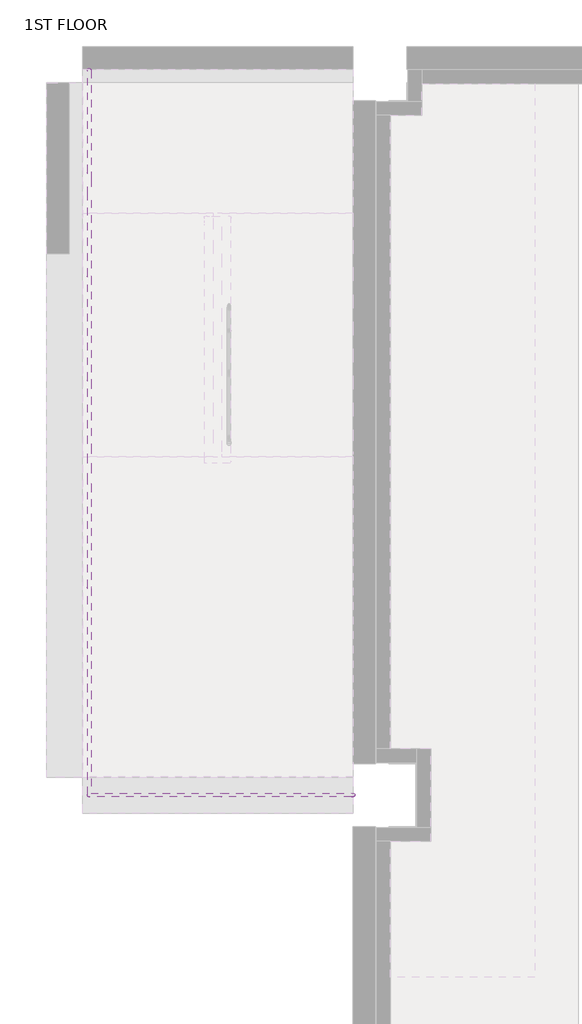
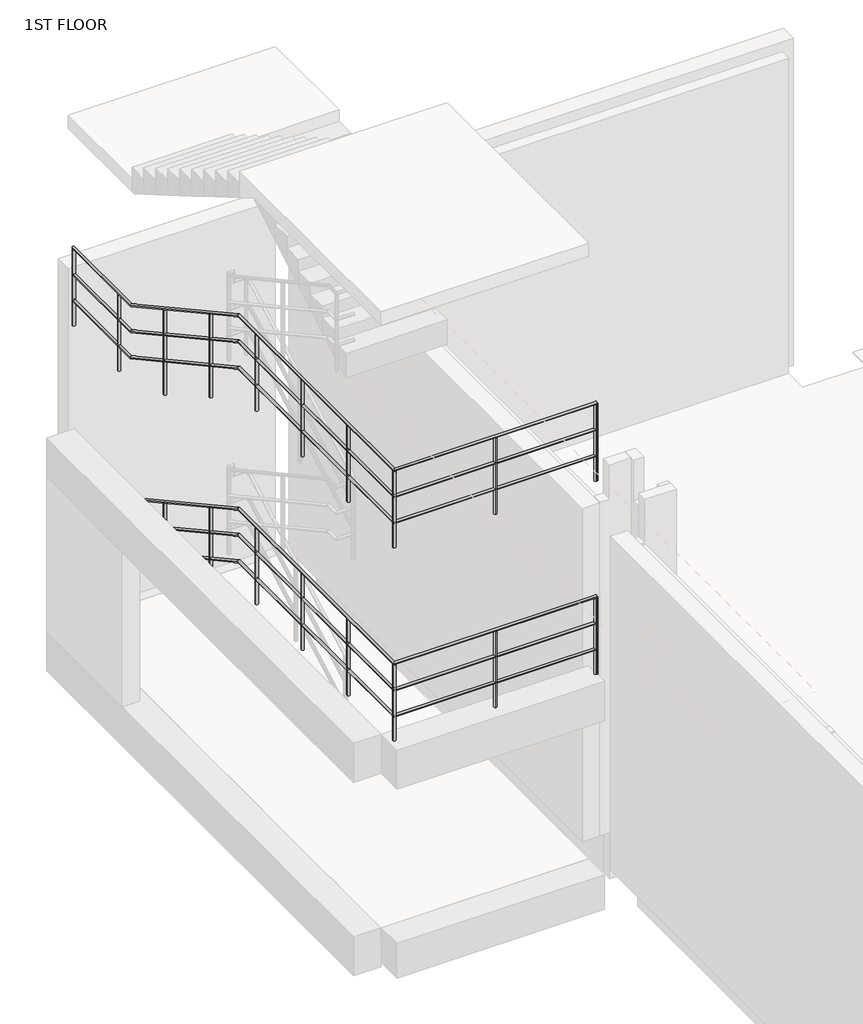
# One storey, part 11 of 15: 2 railings.
"""IFC4 building model written with IfcOpenShell, lengths in millimetres."""

from ifc_helpers import new_model, si_unit, point, frame, frame_2d, origin, place, context, project, spatial, circle_curve, ellipse_curve, trimmed, segment, composite_curve, outline, extrude, element, save
from ifc_brep_helpers import plane_surface, cylinder_surface, advanced_brep

model = new_model("IFC4")

# Units and contexts
model_context = context("Model", 3, world=origin())
ifc_project = project(units=[si_unit("LENGTHUNIT", "METRE", prefix="MILLI")], contexts=[model_context])

# Site, building, storey
site = spatial("IfcSite", under=ifc_project)
building = spatial("IfcBuilding", under=site)
storey = spatial("IfcBuildingStorey", under=building, Name="1ST FLOOR", Elevation=4800.0)

# Railings
placement = place(None, origin())
element("IfcRailing", 1, ObjectType="H_RL_AR_S10_Steel Handrail_H1200_STAIR", at=placement, inside=storey, context=model_context, shape_type="SolidModel", body=[
    advanced_brep(
    [(-3244.0, 50.0, 7291.0), (-3206.0, 50.0, 7291.0), (-3244.0, -1404.865872, 7291.0), (-3206.0, -1404.865872, 7291.0), (-300.0, -8019.0, 8771.0), (-300.0, -7981.0, 8771.0), (-3206.0, -7981.0, 8771.0), (-3244.0, -8019.0, 8771.0), (-3244.0, -4104.865872, 8771.0), (-3206.0, -4104.865872, 8771.0)],
    [
        (0, 1, circle_curve(frame((-3225.0, 50.0, 7291.0), z_axis=(0.0, 1.0, 0.0), x_axis=(1.0, 0.0, 0.0)), 19.0)),
        (1, 0, circle_curve(frame((-3225.0, 50.0, 7291.0), z_axis=(0.0, 1.0, 0.0), x_axis=(1.0, 0.0, 0.0)), 19.0)),
        (0, 2),
        (2, 3, ellipse_curve(frame((-3225.0, -1404.865872, 7291.0), z_axis=(0.0, 0.968736479519294, -0.24809198545814548), x_axis=(0.0, 0.24809198545814504, 0.9687364795192941)), 19.613177, 19.0)),
        (3, 1),
        (3, 2, ellipse_curve(frame((-3225.0, -1404.865872, 7291.0), z_axis=(0.0, 0.968736479519294, -0.24809198545814548), x_axis=(0.0, 0.24809198545814504, 0.9687364795192941)), 19.613177, 19.0)),
        (4, 5, circle_curve(frame((-300.0, -8000.0, 8771.0), z_axis=(1.0, 0.0, 0.0), x_axis=(0.0, 1.0, 0.0)), 19.0)),
        (5, 4, circle_curve(frame((-300.0, -8000.0, 8771.0), z_axis=(1.0, 0.0, 0.0), x_axis=(0.0, 1.0, 0.0)), 19.0)),
        (6, 7, ellipse_curve(frame((-3225.0, -8000.0, 8771.0), z_axis=(0.7071067811865469, -0.707106781186548, 0.0), x_axis=(-0.7071067811865481, -0.7071067811865468, 0.0)), 26.8700577, 19.0)),
        (7, 4),
        (5, 6),
        (7, 6, ellipse_curve(frame((-3225.0, -8000.0, 8771.0), z_axis=(0.7071067811865469, -0.707106781186548, 0.0), x_axis=(-0.7071067811865481, -0.7071067811865468, 0.0)), 26.8700577, 19.0)),
        (2, 8),
        (8, 9, ellipse_curve(frame((-3225.0, -4104.865872, 8771.0), z_axis=(0.0, 0.968736479519294, -0.24809198545814548), x_axis=(0.0, -0.24809198545814592, -0.9687364795192939)), 19.613177, 19.0)),
        (9, 3),
        (9, 8, ellipse_curve(frame((-3225.0, -4104.865872, 8771.0), z_axis=(0.0, 0.968736479519294, -0.24809198545814548), x_axis=(0.0, -0.24809198545814592, -0.9687364795192939)), 19.613177, 19.0)),
        (8, 7),
        (6, 9),
    ],
    [
        plane_surface(frame((-3225.0, 50.0, 7310.0), z_axis=(0.0, 1.0, 0.0), x_axis=(0.0, 0.0, -1.0))),
        cylinder_surface(frame((-3225.0, 50.0, 7291.0), z_axis=(0.0, 1.0, 0.0), x_axis=(1.0, 0.0, 0.0)), 19.0),
        plane_surface(frame((-300.0, -8000.0, 8790.0), z_axis=(1.0, 0.0, 0.0), x_axis=(0.0, 1.0, 0.0))),
        cylinder_surface(frame((-3225.0, -8000.0, 8771.0), z_axis=(-1.0, 0.0, 0.0), x_axis=(0.0, 1.0, 0.0)), 19.0),
        cylinder_surface(frame((-3225.0, -1409.1327588, 7293.3388861), z_axis=(0.0, 0.8769007335028707, -0.4806715131793514), x_axis=(1.0, 0.0, 0.0)), 19.0),
        cylinder_surface(frame((-3225.0, -4100.0, 8771.0), z_axis=(0.0, 1.0, 0.0), x_axis=(1.0, 0.0, 0.0)), 19.0),
    ],
    [
        (0, [[1, 2]]),
        (1, [[-1, 3, 4, 5]]),
        (1, [[-2, -5, 6, -3]]),
        (2, [[7, 8]]),
        (3, [[9, 10, -8, 11]]),
        (3, [[12, -11, -7, -10]]),
        (4, [[-4, 13, 14, 15]]),
        (4, [[-6, -15, 16, -13]]),
        (5, [[-14, 17, -9, 18]]),
        (5, [[-16, -18, -12, -17]]),
    ],
),
    advanced_brep(
    [(-3206.0, 50.0, 6491.0), (-3244.0, 50.0, 6491.0), (-3206.0, -1404.865872, 6491.0), (-3244.0, -1404.865872, 6491.0), (-3206.0, -4104.865872, 7971.0), (-3244.0, -4104.865872, 7971.0), (-3206.0, -7981.0, 7971.0), (-3244.0, -8019.0, 7971.0)],
    [
        (0, 1, circle_curve(frame((-3225.0, 50.0, 6491.0), z_axis=(0.0, 1.0, 0.0), x_axis=(-1.0, 0.0, 0.0)), 19.0)),
        (1, 0, circle_curve(frame((-3225.0, 50.0, 6491.0), z_axis=(0.0, 1.0, 0.0), x_axis=(-1.0, 0.0, 0.0)), 19.0)),
        (0, 2),
        (2, 3, ellipse_curve(frame((-3225.0, -1404.865872, 6491.0), z_axis=(0.0, 0.968736479519294, -0.24809198545814548), x_axis=(0.0, 0.24809198545814504, 0.9687364795192941)), 19.613177, 19.0)),
        (3, 1),
        (3, 2, ellipse_curve(frame((-3225.0, -1404.865872, 6491.0), z_axis=(0.0, 0.968736479519294, -0.24809198545814548), x_axis=(0.0, 0.24809198545814504, 0.9687364795192941)), 19.613177, 19.0)),
        (2, 4),
        (4, 5, ellipse_curve(frame((-3225.0, -4104.865872, 7971.0), z_axis=(0.0, 0.968736479519294, -0.24809198545814548), x_axis=(0.0, -0.24809198545814592, -0.9687364795192939)), 19.613177, 19.0)),
        (5, 3),
        (5, 4, ellipse_curve(frame((-3225.0, -4104.865872, 7971.0), z_axis=(0.0, 0.968736479519294, -0.24809198545814548), x_axis=(0.0, -0.24809198545814592, -0.9687364795192939)), 19.613177, 19.0)),
        (6, 7, ellipse_curve(frame((-3225.0, -8000.0, 7971.0), z_axis=(0.7071067811865464, -0.7071067811865487, 0.0), x_axis=(0.7071067811865487, 0.7071067811865464, 0.0)), 26.8700577, 19.0)),
        (7, 6, ellipse_curve(frame((-3225.0, -8000.0, 7971.0), z_axis=(0.7071067811865464, -0.7071067811865487, 0.0), x_axis=(0.7071067811865487, 0.7071067811865464, 0.0)), 26.8700577, 19.0)),
        (4, 6),
        (7, 5),
    ],
    [
        plane_surface(frame((-3225.0, 50.0, 6510.0), z_axis=(0.0, 1.0, 0.0), x_axis=(0.0, 0.0, -1.0))),
        cylinder_surface(frame((-3225.0, 50.0, 6491.0), z_axis=(0.0, 1.0, 0.0), x_axis=(-1.0, 0.0, 0.0)), 19.0),
        cylinder_surface(frame((-3225.0, -1409.1327588, 6493.3388861), z_axis=(0.0, 0.8769007335028707, -0.4806715131793514), x_axis=(-1.0, 0.0, 0.0)), 19.0),
        plane_surface(frame((-3225.0, -8000.0, 7990.0), z_axis=(0.7071067811865464, -0.7071067811865487, 0.0), x_axis=(0.7071067811865487, 0.7071067811865464, 0.0))),
        cylinder_surface(frame((-3225.0, -4100.0, 7971.0), z_axis=(0.0, 1.0, 0.0), x_axis=(-1.0, 0.0, 0.0)), 19.0),
    ],
    [
        (0, [[1, 2]]),
        (1, [[-1, 3, 4, 5]]),
        (1, [[-2, -5, 6, -3]]),
        (2, [[-4, 7, 8, 9]]),
        (2, [[-6, -9, 10, -7]]),
        (3, [[11, 12]]),
        (4, [[-8, 13, -12, 14]]),
        (4, [[-10, -14, -11, -13]]),
    ],
),
    advanced_brep(
    [(-3206.0, -7981.0, 7971.0), (-3244.0, -8019.0, 7971.0), (-300.0, -7981.0, 7971.0), (-300.0, -8019.0, 7971.0)],
    [
        (0, 1, ellipse_curve(frame((-3225.0, -8000.0, 7971.0), z_axis=(-0.7071067811865464, 0.7071067811865487, 0.0), x_axis=(-0.7071067811865487, -0.7071067811865464, 0.0)), 26.8700577, 19.0)),
        (1, 0, ellipse_curve(frame((-3225.0, -8000.0, 7971.0), z_axis=(-0.7071067811865464, 0.7071067811865487, 0.0), x_axis=(-0.7071067811865487, -0.7071067811865464, 0.0)), 26.8700577, 19.0)),
        (2, 3, circle_curve(frame((-300.0, -8000.0, 7971.0), z_axis=(1.0, 0.0, 0.0), x_axis=(0.0, -1.0, 0.0)), 19.0)),
        (3, 2, circle_curve(frame((-300.0, -8000.0, 7971.0), z_axis=(1.0, 0.0, 0.0), x_axis=(0.0, -1.0, 0.0)), 19.0)),
        (0, 2),
        (3, 1),
    ],
    [
        plane_surface(frame((-3225.0, -8000.0, 7990.0), z_axis=(-0.7071067811865464, 0.7071067811865487, 0.0), x_axis=(0.7071067811865487, 0.7071067811865464, 0.0))),
        plane_surface(frame((-300.0, -8000.0, 7990.0), z_axis=(1.0, 0.0, 0.0), x_axis=(0.0, 1.0, 0.0))),
        cylinder_surface(frame((-3225.0, -8000.0, 7971.0), z_axis=(-1.0, 0.0, 0.0), x_axis=(0.0, -1.0, 0.0)), 19.0),
    ],
    [
        (0, [[1, 2]]),
        (1, [[3, 4]]),
        (2, [[-1, 5, -4, 6]]),
        (2, [[-2, -6, -3, -5]]),
    ],
),
    advanced_brep(
    [(-3206.0, 50.0, 6891.0), (-3244.0, 50.0, 6891.0), (-3206.0, -1404.865872, 6891.0), (-3244.0, -1404.865872, 6891.0), (-3206.0, -4104.865872, 8371.0), (-3244.0, -4104.865872, 8371.0), (-3206.0, -7981.0, 8371.0), (-3244.0, -8019.0, 8371.0)],
    [
        (0, 1, circle_curve(frame((-3225.0, 50.0, 6891.0), z_axis=(0.0, 1.0, 0.0), x_axis=(-1.0, 0.0, 0.0)), 19.0)),
        (1, 0, circle_curve(frame((-3225.0, 50.0, 6891.0), z_axis=(0.0, 1.0, 0.0), x_axis=(-1.0, 0.0, 0.0)), 19.0)),
        (0, 2),
        (2, 3, ellipse_curve(frame((-3225.0, -1404.865872, 6891.0), z_axis=(0.0, 0.968736479519294, -0.24809198545814548), x_axis=(0.0, 0.24809198545814504, 0.9687364795192941)), 19.613177, 19.0)),
        (3, 1),
        (3, 2, ellipse_curve(frame((-3225.0, -1404.865872, 6891.0), z_axis=(0.0, 0.968736479519294, -0.24809198545814548), x_axis=(0.0, 0.24809198545814504, 0.9687364795192941)), 19.613177, 19.0)),
        (2, 4),
        (4, 5, ellipse_curve(frame((-3225.0, -4104.865872, 8371.0), z_axis=(0.0, 0.968736479519294, -0.24809198545814548), x_axis=(0.0, -0.24809198545814592, -0.9687364795192939)), 19.613177, 19.0)),
        (5, 3),
        (5, 4, ellipse_curve(frame((-3225.0, -4104.865872, 8371.0), z_axis=(0.0, 0.968736479519294, -0.24809198545814548), x_axis=(0.0, -0.24809198545814592, -0.9687364795192939)), 19.613177, 19.0)),
        (6, 7, ellipse_curve(frame((-3225.0, -8000.0, 8371.0), z_axis=(0.7071067811865464, -0.7071067811865487, 0.0), x_axis=(0.7071067811865487, 0.7071067811865464, 0.0)), 26.8700577, 19.0)),
        (7, 6, ellipse_curve(frame((-3225.0, -8000.0, 8371.0), z_axis=(0.7071067811865464, -0.7071067811865487, 0.0), x_axis=(0.7071067811865487, 0.7071067811865464, 0.0)), 26.8700577, 19.0)),
        (4, 6),
        (7, 5),
    ],
    [
        plane_surface(frame((-3225.0, 50.0, 6910.0), z_axis=(0.0, 1.0, 0.0), x_axis=(0.0, 0.0, -1.0))),
        cylinder_surface(frame((-3225.0, 50.0, 6891.0), z_axis=(0.0, 1.0, 0.0), x_axis=(-1.0, 0.0, 0.0)), 19.0),
        cylinder_surface(frame((-3225.0, -1409.1327588, 6893.3388861), z_axis=(0.0, 0.8769007335028707, -0.4806715131793514), x_axis=(-1.0, 0.0, 0.0)), 19.0),
        plane_surface(frame((-3225.0, -8000.0, 8390.0), z_axis=(0.7071067811865464, -0.7071067811865487, 0.0), x_axis=(0.7071067811865487, 0.7071067811865464, 0.0))),
        cylinder_surface(frame((-3225.0, -4100.0, 8371.0), z_axis=(0.0, 1.0, 0.0), x_axis=(-1.0, 0.0, 0.0)), 19.0),
    ],
    [
        (0, [[1, 2]]),
        (1, [[-1, 3, 4, 5]]),
        (1, [[-2, -5, 6, -3]]),
        (2, [[-4, 7, 8, 9]]),
        (2, [[-6, -9, 10, -7]]),
        (3, [[11, 12]]),
        (4, [[-8, 13, -12, 14]]),
        (4, [[-10, -14, -11, -13]]),
    ],
),
    advanced_brep(
    [(-3206.0, -7981.0, 8371.0), (-3244.0, -8019.0, 8371.0), (-300.0, -7981.0, 8371.0), (-300.0, -8019.0, 8371.0)],
    [
        (0, 1, ellipse_curve(frame((-3225.0, -8000.0, 8371.0), z_axis=(-0.7071067811865464, 0.7071067811865487, 0.0), x_axis=(-0.7071067811865487, -0.7071067811865464, 0.0)), 26.8700577, 19.0)),
        (1, 0, ellipse_curve(frame((-3225.0, -8000.0, 8371.0), z_axis=(-0.7071067811865464, 0.7071067811865487, 0.0), x_axis=(-0.7071067811865487, -0.7071067811865464, 0.0)), 26.8700577, 19.0)),
        (2, 3, circle_curve(frame((-300.0, -8000.0, 8371.0), z_axis=(1.0, 0.0, 0.0), x_axis=(0.0, -1.0, 0.0)), 19.0)),
        (3, 2, circle_curve(frame((-300.0, -8000.0, 8371.0), z_axis=(1.0, 0.0, 0.0), x_axis=(0.0, -1.0, 0.0)), 19.0)),
        (0, 2),
        (3, 1),
    ],
    [
        plane_surface(frame((-3225.0, -8000.0, 8390.0), z_axis=(-0.7071067811865464, 0.7071067811865487, 0.0), x_axis=(0.7071067811865487, 0.7071067811865464, 0.0))),
        plane_surface(frame((-300.0, -8000.0, 8390.0), z_axis=(1.0, 0.0, 0.0), x_axis=(0.0, 1.0, 0.0))),
        cylinder_surface(frame((-3225.0, -8000.0, 8371.0), z_axis=(-1.0, 0.0, 0.0), x_axis=(0.0, -1.0, 0.0)), 19.0),
    ],
    [
        (0, [[1, 2]]),
        (1, [[3, 4]]),
        (2, [[-1, 5, -4, 6]]),
        (2, [[-2, -6, -3, -5]]),
    ],
),
    extrude(outline(composite_curve([segment(trimmed(circle_curve(frame_2d((-300.0, -8000.0)), 21.2), [point((-300.0, -7978.8))], [point((-300.0, -8021.2))], False, "CARTESIAN"), True, "CONTINUOUS"), segment(trimmed(circle_curve(frame_2d((-300.0, -8000.0)), 21.2), [point((-300.0, -8021.2))], [point((-300.0, -7978.8))], False, "CARTESIAN"), True, "CONTINUOUS")], self_intersect=False)), frame((0.0, 0.0, 7590.0), z_axis=(0.0, 0.0, 1.0), x_axis=(1.0, 0.0, 0.0)), (0.0, 0.0, 1.0), 1162.0),
    extrude(outline(composite_curve([segment(trimmed(circle_curve(frame_2d((-1762.5, -8000.0)), 21.2), [point((-1762.5, -7978.8))], [point((-1762.5, -8021.2))], False, "CARTESIAN"), True, "CONTINUOUS"), segment(trimmed(circle_curve(frame_2d((-1762.5, -8000.0)), 21.2), [point((-1762.5, -8021.2))], [point((-1762.5, -7978.8))], False, "CARTESIAN"), True, "CONTINUOUS")], self_intersect=False)), frame((0.0, 0.0, 7590.0), z_axis=(0.0, 0.0, 1.0), x_axis=(1.0, 0.0, 0.0)), (0.0, 0.0, 1.0), 1162.0),
    extrude(outline(composite_curve([segment(trimmed(circle_curve(frame_2d((-3225.0, -8000.0)), 21.2), [point((-3203.8, -8000.0))], [point((-3246.2, -8000.0))], False, "CARTESIAN"), True, "CONTINUOUS"), segment(trimmed(circle_curve(frame_2d((-3225.0, -8000.0)), 21.2), [point((-3246.2, -8000.0))], [point((-3203.8, -8000.0))], False, "CARTESIAN"), True, "CONTINUOUS")], self_intersect=False)), frame((0.0, 0.0, 7590.0), z_axis=(0.0, 0.0, 1.0), x_axis=(1.0, 0.0, 0.0)), (0.0, 0.0, 1.0), 1162.0),
    extrude(outline(composite_curve([segment(trimmed(circle_curve(frame_2d((-3225.0, -6850.0)), 21.2), [point((-3203.8, -6850.0))], [point((-3246.2, -6850.0))], False, "CARTESIAN"), True, "CONTINUOUS"), segment(trimmed(circle_curve(frame_2d((-3225.0, -6850.0)), 21.2), [point((-3246.2, -6850.0))], [point((-3203.8, -6850.0))], False, "CARTESIAN"), True, "CONTINUOUS")], self_intersect=False)), frame((0.0, 0.0, 7590.0), z_axis=(0.0, 0.0, 1.0), x_axis=(1.0, 0.0, 0.0)), (0.0, 0.0, 1.0), 1162.0),
    extrude(outline(composite_curve([segment(trimmed(circle_curve(frame_2d((-3225.0, -5700.0)), 21.2), [point((-3203.8, -5700.0))], [point((-3246.2, -5700.0))], False, "CARTESIAN"), True, "CONTINUOUS"), segment(trimmed(circle_curve(frame_2d((-3225.0, -5700.0)), 21.2), [point((-3246.2, -5700.0))], [point((-3203.8, -5700.0))], False, "CARTESIAN"), True, "CONTINUOUS")], self_intersect=False)), frame((0.0, 0.0, 7590.0), z_axis=(0.0, 0.0, 1.0), x_axis=(1.0, 0.0, 0.0)), (0.0, 0.0, 1.0), 1162.0),
    extrude(outline(composite_curve([segment(trimmed(circle_curve(frame_2d((-3225.0, -4550.0)), 21.2), [point((-3203.8, -4550.0))], [point((-3246.2, -4550.0))], False, "CARTESIAN"), True, "CONTINUOUS"), segment(trimmed(circle_curve(frame_2d((-3225.0, -4550.0)), 21.2), [point((-3246.2, -4550.0))], [point((-3203.8, -4550.0))], False, "CARTESIAN"), True, "CONTINUOUS")], self_intersect=False)), frame((0.0, 0.0, 7590.0), z_axis=(0.0, 0.0, 1.0), x_axis=(1.0, 0.0, 0.0)), (0.0, 0.0, 1.0), 1162.0),
    advanced_brep(
    [(-3246.2, -3400.0, 8362.9618588), (-3246.2, -3400.0, 7096.6666667), (-3203.8, -3400.0, 7096.6666667), (-3203.8, -3400.0, 8362.9618588)],
    [
        (0, 1),
        (1, 2, circle_curve(frame((-3225.0, -3400.0, 7096.6666667), z_axis=(0.0, 0.0, 1.0), x_axis=(1.0, 0.0, 0.0)), 21.2)),
        (2, 3),
        (3, 0, ellipse_curve(frame((-3225.0, -3400.0, 8362.9618588), z_axis=(0.0, -0.4806715131793532, -0.8769007335028697), x_axis=(0.0, -0.8769007335028696, 0.4806715131793532)), 24.1760546, 21.2)),
        (0, 3, ellipse_curve(frame((-3225.0, -3400.0, 8362.9618588), z_axis=(0.0, -0.4806715131793532, -0.8769007335028697), x_axis=(0.0, -0.8769007335028696, 0.4806715131793532)), 24.1760546, 21.2)),
        (2, 1, circle_curve(frame((-3225.0, -3400.0, 7096.6666667), z_axis=(0.0, 0.0, 1.0), x_axis=(1.0, 0.0, 0.0)), 21.2)),
    ],
    [
        cylinder_surface(frame((-3225.0, -3400.0, 6996.6666667), z_axis=(0.0, 0.0, 1.0), x_axis=(1.0, 0.0, 0.0)), 21.2),
        plane_surface(frame((-3200.0, -3425.0, 8376.6655625), z_axis=(0.0, 0.4806715131793532, 0.8769007335028697), x_axis=(-1.0, 0.0, 0.0))),
        plane_surface(frame((-3200.0, -3375.0, 7096.6666667), z_axis=(0.0, 0.0, -1.0), x_axis=(-1.0, 0.0, 0.0))),
    ],
    [
        (0, [[1, 2, 3, 4]]),
        (0, [[-1, 5, -3, 6]]),
        (1, [[-4, -5]]),
        (2, [[-2, -6]]),
    ],
),
    advanced_brep(
    [(-3246.2, -2250.0, 7732.5914885), (-3246.2, -2250.0, 6438.8888889), (-3203.8, -2250.0, 6438.8888889), (-3203.8, -2250.0, 7732.5914885)],
    [
        (0, 1),
        (1, 2, circle_curve(frame((-3225.0, -2250.0, 6438.8888889), z_axis=(0.0, 0.0, 1.0), x_axis=(1.0, 0.0, 0.0)), 21.2)),
        (2, 3),
        (3, 0, ellipse_curve(frame((-3225.0, -2250.0, 7732.5914885), z_axis=(0.0, -0.4806715131793496, -0.8769007335028717), x_axis=(0.0, -0.8769007335028718, 0.4806715131793496)), 24.1760546, 21.2)),
        (0, 3, ellipse_curve(frame((-3225.0, -2250.0, 7732.5914885), z_axis=(0.0, -0.4806715131793496, -0.8769007335028717), x_axis=(0.0, -0.8769007335028718, 0.4806715131793496)), 24.1760546, 21.2)),
        (2, 1, circle_curve(frame((-3225.0, -2250.0, 6438.8888889), z_axis=(0.0, 0.0, 1.0), x_axis=(1.0, 0.0, 0.0)), 21.2)),
    ],
    [
        cylinder_surface(frame((-3225.0, -2250.0, 6338.8888889), z_axis=(0.0, 0.0, 1.0), x_axis=(1.0, 0.0, 0.0)), 21.2),
        plane_surface(frame((-3200.0, -2275.0, 7746.2951922), z_axis=(0.0, 0.4806715131793496, 0.8769007335028717), x_axis=(-1.0, 0.0, 0.0))),
        plane_surface(frame((-3200.0, -2225.0, 6438.8888889), z_axis=(0.0, 0.0, -1.0), x_axis=(-1.0, 0.0, 0.0))),
    ],
    [
        (0, [[1, 2, 3, 4]]),
        (0, [[-1, 5, -3, 6]]),
        (1, [[-4, -5]]),
        (2, [[-2, -6]]),
    ],
),
    extrude(outline(composite_curve([segment(trimmed(circle_curve(frame_2d((-3225.0, -1100.0)), 21.2), [point((-3203.8, -1100.0))], [point((-3246.2, -1100.0))], False, "CARTESIAN"), True, "CONTINUOUS"), segment(trimmed(circle_curve(frame_2d((-3225.0, -1100.0)), 21.2), [point((-3246.2, -1100.0))], [point((-3203.8, -1100.0))], False, "CARTESIAN"), True, "CONTINUOUS")], self_intersect=False)), frame((0.0, 0.0, 6110.0), z_axis=(0.0, 0.0, 1.0), x_axis=(1.0, 0.0, 0.0)), (0.0, 0.0, 1.0), 1162.0),
    extrude(outline(composite_curve([segment(trimmed(circle_curve(frame_2d((-312.5, -8000.0)), 21.2), [point((-312.5, -7978.8))], [point((-312.5, -8021.2))], False, "CARTESIAN"), True, "CONTINUOUS"), segment(trimmed(circle_curve(frame_2d((-312.5, -8000.0)), 21.2), [point((-312.5, -8021.2))], [point((-312.5, -7978.8))], False, "CARTESIAN"), True, "CONTINUOUS")], self_intersect=False)), frame((0.0, 0.0, 7590.0), z_axis=(0.0, 0.0, 1.0), x_axis=(1.0, 0.0, 0.0)), (0.0, 0.0, 1.0), 1162.0),
    extrude(outline(composite_curve([segment(trimmed(circle_curve(frame_2d((-3225.0, 37.5)), 21.2), [point((-3203.8, 37.5))], [point((-3246.2, 37.5))], False, "CARTESIAN"), True, "CONTINUOUS"), segment(trimmed(circle_curve(frame_2d((-3225.0, 37.5)), 21.2), [point((-3246.2, 37.5))], [point((-3203.8, 37.5))], False, "CARTESIAN"), True, "CONTINUOUS")], self_intersect=False)), frame((0.0, 0.0, 6110.0), z_axis=(0.0, 0.0, 1.0), x_axis=(1.0, 0.0, 0.0)), (0.0, 0.0, 1.0), 1162.0),
])
element("IfcRailing", 2, ObjectType="H_RL_AR_S10_Steel Handrail_H1200_STAIR", at=placement, inside=storey, context=model_context, shape_type="SolidModel", body=[
    advanced_brep(
    [(-3244.0, 50.0, 10251.0), (-3206.0, 50.0, 10251.0), (-3244.0, -1404.865872, 10251.0), (-3206.0, -1404.865872, 10251.0), (-300.0, -8019.0, 11731.0), (-300.0, -7981.0, 11731.0), (-3206.0, -7981.0, 11731.0), (-3244.0, -8019.0, 11731.0), (-3244.0, -4104.865872, 11731.0), (-3206.0, -4104.865872, 11731.0)],
    [
        (0, 1, circle_curve(frame((-3225.0, 50.0, 10251.0), z_axis=(0.0, 1.0, 0.0), x_axis=(1.0, 0.0, 0.0)), 19.0)),
        (1, 0, circle_curve(frame((-3225.0, 50.0, 10251.0), z_axis=(0.0, 1.0, 0.0), x_axis=(1.0, 0.0, 0.0)), 19.0)),
        (0, 2),
        (2, 3, ellipse_curve(frame((-3225.0, -1404.865872, 10251.0), z_axis=(0.0, 0.968736479519294, -0.24809198545814548), x_axis=(0.0, 0.24809198545814504, 0.9687364795192941)), 19.613177, 19.0)),
        (3, 1),
        (3, 2, ellipse_curve(frame((-3225.0, -1404.865872, 10251.0), z_axis=(0.0, 0.968736479519294, -0.24809198545814548), x_axis=(0.0, 0.24809198545814504, 0.9687364795192941)), 19.613177, 19.0)),
        (4, 5, circle_curve(frame((-300.0, -8000.0, 11731.0), z_axis=(1.0, 0.0, 0.0), x_axis=(0.0, 1.0, 0.0)), 19.0)),
        (5, 4, circle_curve(frame((-300.0, -8000.0, 11731.0), z_axis=(1.0, 0.0, 0.0), x_axis=(0.0, 1.0, 0.0)), 19.0)),
        (6, 7, ellipse_curve(frame((-3225.0, -8000.0, 11731.0), z_axis=(0.7071067811865469, -0.707106781186548, 0.0), x_axis=(-0.7071067811865481, -0.7071067811865468, 0.0)), 26.8700577, 19.0)),
        (7, 4),
        (5, 6),
        (7, 6, ellipse_curve(frame((-3225.0, -8000.0, 11731.0), z_axis=(0.7071067811865469, -0.707106781186548, 0.0), x_axis=(-0.7071067811865481, -0.7071067811865468, 0.0)), 26.8700577, 19.0)),
        (2, 8),
        (8, 9, ellipse_curve(frame((-3225.0, -4104.865872, 11731.0), z_axis=(0.0, 0.968736479519294, -0.24809198545814548), x_axis=(0.0, -0.24809198545814592, -0.9687364795192939)), 19.613177, 19.0)),
        (9, 3),
        (9, 8, ellipse_curve(frame((-3225.0, -4104.865872, 11731.0), z_axis=(0.0, 0.968736479519294, -0.24809198545814548), x_axis=(0.0, -0.24809198545814592, -0.9687364795192939)), 19.613177, 19.0)),
        (8, 7),
        (6, 9),
    ],
    [
        plane_surface(frame((-3225.0, 50.0, 10270.0), z_axis=(0.0, 1.0, 0.0), x_axis=(0.0, 0.0, -1.0))),
        cylinder_surface(frame((-3225.0, 50.0, 10251.0), z_axis=(0.0, 1.0, 0.0), x_axis=(1.0, 0.0, 0.0)), 19.0),
        plane_surface(frame((-300.0, -8000.0, 11750.0), z_axis=(1.0, 0.0, 0.0), x_axis=(0.0, 1.0, 0.0))),
        cylinder_surface(frame((-3225.0, -8000.0, 11731.0), z_axis=(-1.0, 0.0, 0.0), x_axis=(0.0, 1.0, 0.0)), 19.0),
        cylinder_surface(frame((-3225.0, -1409.1327588, 10253.3388861), z_axis=(0.0, 0.8769007335028707, -0.4806715131793514), x_axis=(1.0, 0.0, 0.0)), 19.0),
        cylinder_surface(frame((-3225.0, -4100.0, 11731.0), z_axis=(0.0, 1.0, 0.0), x_axis=(1.0, 0.0, 0.0)), 19.0),
    ],
    [
        (0, [[1, 2]]),
        (1, [[-1, 3, 4, 5]]),
        (1, [[-2, -5, 6, -3]]),
        (2, [[7, 8]]),
        (3, [[9, 10, -8, 11]]),
        (3, [[12, -11, -7, -10]]),
        (4, [[-4, 13, 14, 15]]),
        (4, [[-6, -15, 16, -13]]),
        (5, [[-14, 17, -9, 18]]),
        (5, [[-16, -18, -12, -17]]),
    ],
),
    advanced_brep(
    [(-3206.0, 50.0, 9451.0), (-3244.0, 50.0, 9451.0), (-3206.0, -1404.865872, 9451.0), (-3244.0, -1404.865872, 9451.0), (-3206.0, -4104.865872, 10931.0), (-3244.0, -4104.865872, 10931.0), (-3206.0, -7981.0, 10931.0), (-3244.0, -8019.0, 10931.0)],
    [
        (0, 1, circle_curve(frame((-3225.0, 50.0, 9451.0), z_axis=(0.0, 1.0, 0.0), x_axis=(-1.0, 0.0, 0.0)), 19.0)),
        (1, 0, circle_curve(frame((-3225.0, 50.0, 9451.0), z_axis=(0.0, 1.0, 0.0), x_axis=(-1.0, 0.0, 0.0)), 19.0)),
        (0, 2),
        (2, 3, ellipse_curve(frame((-3225.0, -1404.865872, 9451.0), z_axis=(0.0, 0.968736479519294, -0.24809198545814548), x_axis=(0.0, 0.24809198545814504, 0.9687364795192941)), 19.613177, 19.0)),
        (3, 1),
        (3, 2, ellipse_curve(frame((-3225.0, -1404.865872, 9451.0), z_axis=(0.0, 0.968736479519294, -0.24809198545814548), x_axis=(0.0, 0.24809198545814504, 0.9687364795192941)), 19.613177, 19.0)),
        (2, 4),
        (4, 5, ellipse_curve(frame((-3225.0, -4104.865872, 10931.0), z_axis=(0.0, 0.968736479519294, -0.24809198545814548), x_axis=(0.0, -0.24809198545814592, -0.9687364795192939)), 19.613177, 19.0)),
        (5, 3),
        (5, 4, ellipse_curve(frame((-3225.0, -4104.865872, 10931.0), z_axis=(0.0, 0.968736479519294, -0.24809198545814548), x_axis=(0.0, -0.24809198545814592, -0.9687364795192939)), 19.613177, 19.0)),
        (6, 7, ellipse_curve(frame((-3225.0, -8000.0, 10931.0), z_axis=(0.7071067811865464, -0.7071067811865487, 0.0), x_axis=(0.7071067811865487, 0.7071067811865464, 0.0)), 26.8700577, 19.0)),
        (7, 6, ellipse_curve(frame((-3225.0, -8000.0, 10931.0), z_axis=(0.7071067811865464, -0.7071067811865487, 0.0), x_axis=(0.7071067811865487, 0.7071067811865464, 0.0)), 26.8700577, 19.0)),
        (4, 6),
        (7, 5),
    ],
    [
        plane_surface(frame((-3225.0, 50.0, 9470.0), z_axis=(0.0, 1.0, 0.0), x_axis=(0.0, 0.0, -1.0))),
        cylinder_surface(frame((-3225.0, 50.0, 9451.0), z_axis=(0.0, 1.0, 0.0), x_axis=(-1.0, 0.0, 0.0)), 19.0),
        cylinder_surface(frame((-3225.0, -1409.1327588, 9453.3388861), z_axis=(0.0, 0.8769007335028707, -0.4806715131793514), x_axis=(-1.0, 0.0, 0.0)), 19.0),
        plane_surface(frame((-3225.0, -8000.0, 10950.0), z_axis=(0.7071067811865464, -0.7071067811865487, 0.0), x_axis=(0.7071067811865487, 0.7071067811865464, 0.0))),
        cylinder_surface(frame((-3225.0, -4100.0, 10931.0), z_axis=(0.0, 1.0, 0.0), x_axis=(-1.0, 0.0, 0.0)), 19.0),
    ],
    [
        (0, [[1, 2]]),
        (1, [[-1, 3, 4, 5]]),
        (1, [[-2, -5, 6, -3]]),
        (2, [[-4, 7, 8, 9]]),
        (2, [[-6, -9, 10, -7]]),
        (3, [[11, 12]]),
        (4, [[-8, 13, -12, 14]]),
        (4, [[-10, -14, -11, -13]]),
    ],
),
    advanced_brep(
    [(-3206.0, -7981.0, 10931.0), (-3244.0, -8019.0, 10931.0), (-300.0, -7981.0, 10931.0), (-300.0, -8019.0, 10931.0)],
    [
        (0, 1, ellipse_curve(frame((-3225.0, -8000.0, 10931.0), z_axis=(-0.7071067811865464, 0.7071067811865487, 0.0), x_axis=(-0.7071067811865487, -0.7071067811865464, 0.0)), 26.8700577, 19.0)),
        (1, 0, ellipse_curve(frame((-3225.0, -8000.0, 10931.0), z_axis=(-0.7071067811865464, 0.7071067811865487, 0.0), x_axis=(-0.7071067811865487, -0.7071067811865464, 0.0)), 26.8700577, 19.0)),
        (2, 3, circle_curve(frame((-300.0, -8000.0, 10931.0), z_axis=(1.0, 0.0, 0.0), x_axis=(0.0, -1.0, 0.0)), 19.0)),
        (3, 2, circle_curve(frame((-300.0, -8000.0, 10931.0), z_axis=(1.0, 0.0, 0.0), x_axis=(0.0, -1.0, 0.0)), 19.0)),
        (0, 2),
        (3, 1),
    ],
    [
        plane_surface(frame((-3225.0, -8000.0, 10950.0), z_axis=(-0.7071067811865464, 0.7071067811865487, 0.0), x_axis=(0.7071067811865487, 0.7071067811865464, 0.0))),
        plane_surface(frame((-300.0, -8000.0, 10950.0), z_axis=(1.0, 0.0, 0.0), x_axis=(0.0, 1.0, 0.0))),
        cylinder_surface(frame((-3225.0, -8000.0, 10931.0), z_axis=(-1.0, 0.0, 0.0), x_axis=(0.0, -1.0, 0.0)), 19.0),
    ],
    [
        (0, [[1, 2]]),
        (1, [[3, 4]]),
        (2, [[-1, 5, -4, 6]]),
        (2, [[-2, -6, -3, -5]]),
    ],
),
    advanced_brep(
    [(-3206.0, 50.0, 9851.0), (-3244.0, 50.0, 9851.0), (-3206.0, -1404.865872, 9851.0), (-3244.0, -1404.865872, 9851.0), (-3206.0, -4104.865872, 11331.0), (-3244.0, -4104.865872, 11331.0), (-3206.0, -7981.0, 11331.0), (-3244.0, -8019.0, 11331.0)],
    [
        (0, 1, circle_curve(frame((-3225.0, 50.0, 9851.0), z_axis=(0.0, 1.0, 0.0), x_axis=(-1.0, 0.0, 0.0)), 19.0)),
        (1, 0, circle_curve(frame((-3225.0, 50.0, 9851.0), z_axis=(0.0, 1.0, 0.0), x_axis=(-1.0, 0.0, 0.0)), 19.0)),
        (0, 2),
        (2, 3, ellipse_curve(frame((-3225.0, -1404.865872, 9851.0), z_axis=(0.0, 0.968736479519294, -0.24809198545814548), x_axis=(0.0, 0.24809198545814504, 0.9687364795192941)), 19.613177, 19.0)),
        (3, 1),
        (3, 2, ellipse_curve(frame((-3225.0, -1404.865872, 9851.0), z_axis=(0.0, 0.968736479519294, -0.24809198545814548), x_axis=(0.0, 0.24809198545814504, 0.9687364795192941)), 19.613177, 19.0)),
        (2, 4),
        (4, 5, ellipse_curve(frame((-3225.0, -4104.865872, 11331.0), z_axis=(0.0, 0.968736479519294, -0.24809198545814548), x_axis=(0.0, -0.24809198545814592, -0.9687364795192939)), 19.613177, 19.0)),
        (5, 3),
        (5, 4, ellipse_curve(frame((-3225.0, -4104.865872, 11331.0), z_axis=(0.0, 0.968736479519294, -0.24809198545814548), x_axis=(0.0, -0.24809198545814592, -0.9687364795192939)), 19.613177, 19.0)),
        (6, 7, ellipse_curve(frame((-3225.0, -8000.0, 11331.0), z_axis=(0.7071067811865464, -0.7071067811865487, 0.0), x_axis=(0.7071067811865487, 0.7071067811865464, 0.0)), 26.8700577, 19.0)),
        (7, 6, ellipse_curve(frame((-3225.0, -8000.0, 11331.0), z_axis=(0.7071067811865464, -0.7071067811865487, 0.0), x_axis=(0.7071067811865487, 0.7071067811865464, 0.0)), 26.8700577, 19.0)),
        (4, 6),
        (7, 5),
    ],
    [
        plane_surface(frame((-3225.0, 50.0, 9870.0), z_axis=(0.0, 1.0, 0.0), x_axis=(0.0, 0.0, -1.0))),
        cylinder_surface(frame((-3225.0, 50.0, 9851.0), z_axis=(0.0, 1.0, 0.0), x_axis=(-1.0, 0.0, 0.0)), 19.0),
        cylinder_surface(frame((-3225.0, -1409.1327588, 9853.3388861), z_axis=(0.0, 0.8769007335028707, -0.4806715131793514), x_axis=(-1.0, 0.0, 0.0)), 19.0),
        plane_surface(frame((-3225.0, -8000.0, 11350.0), z_axis=(0.7071067811865464, -0.7071067811865487, 0.0), x_axis=(0.7071067811865487, 0.7071067811865464, 0.0))),
        cylinder_surface(frame((-3225.0, -4100.0, 11331.0), z_axis=(0.0, 1.0, 0.0), x_axis=(-1.0, 0.0, 0.0)), 19.0),
    ],
    [
        (0, [[1, 2]]),
        (1, [[-1, 3, 4, 5]]),
        (1, [[-2, -5, 6, -3]]),
        (2, [[-4, 7, 8, 9]]),
        (2, [[-6, -9, 10, -7]]),
        (3, [[11, 12]]),
        (4, [[-8, 13, -12, 14]]),
        (4, [[-10, -14, -11, -13]]),
    ],
),
    advanced_brep(
    [(-3206.0, -7981.0, 11331.0), (-3244.0, -8019.0, 11331.0), (-300.0, -7981.0, 11331.0), (-300.0, -8019.0, 11331.0)],
    [
        (0, 1, ellipse_curve(frame((-3225.0, -8000.0, 11331.0), z_axis=(-0.7071067811865464, 0.7071067811865487, 0.0), x_axis=(-0.7071067811865487, -0.7071067811865464, 0.0)), 26.8700577, 19.0)),
        (1, 0, ellipse_curve(frame((-3225.0, -8000.0, 11331.0), z_axis=(-0.7071067811865464, 0.7071067811865487, 0.0), x_axis=(-0.7071067811865487, -0.7071067811865464, 0.0)), 26.8700577, 19.0)),
        (2, 3, circle_curve(frame((-300.0, -8000.0, 11331.0), z_axis=(1.0, 0.0, 0.0), x_axis=(0.0, -1.0, 0.0)), 19.0)),
        (3, 2, circle_curve(frame((-300.0, -8000.0, 11331.0), z_axis=(1.0, 0.0, 0.0), x_axis=(0.0, -1.0, 0.0)), 19.0)),
        (0, 2),
        (3, 1),
    ],
    [
        plane_surface(frame((-3225.0, -8000.0, 11350.0), z_axis=(-0.7071067811865464, 0.7071067811865487, 0.0), x_axis=(0.7071067811865487, 0.7071067811865464, 0.0))),
        plane_surface(frame((-300.0, -8000.0, 11350.0), z_axis=(1.0, 0.0, 0.0), x_axis=(0.0, 1.0, 0.0))),
        cylinder_surface(frame((-3225.0, -8000.0, 11331.0), z_axis=(-1.0, 0.0, 0.0), x_axis=(0.0, -1.0, 0.0)), 19.0),
    ],
    [
        (0, [[1, 2]]),
        (1, [[3, 4]]),
        (2, [[-1, 5, -4, 6]]),
        (2, [[-2, -6, -3, -5]]),
    ],
),
    extrude(outline(composite_curve([segment(trimmed(circle_curve(frame_2d((-300.0, -8000.0)), 21.2), [point((-300.0, -7978.8))], [point((-300.0, -8021.2))], False, "CARTESIAN"), True, "CONTINUOUS"), segment(trimmed(circle_curve(frame_2d((-300.0, -8000.0)), 21.2), [point((-300.0, -8021.2))], [point((-300.0, -7978.8))], False, "CARTESIAN"), True, "CONTINUOUS")], self_intersect=False)), frame((0.0, 0.0, 10550.0), z_axis=(0.0, 0.0, 1.0), x_axis=(1.0, 0.0, 0.0)), (0.0, 0.0, 1.0), 1162.0),
    extrude(outline(composite_curve([segment(trimmed(circle_curve(frame_2d((-1762.5, -8000.0)), 21.2), [point((-1762.5, -7978.8))], [point((-1762.5, -8021.2))], False, "CARTESIAN"), True, "CONTINUOUS"), segment(trimmed(circle_curve(frame_2d((-1762.5, -8000.0)), 21.2), [point((-1762.5, -8021.2))], [point((-1762.5, -7978.8))], False, "CARTESIAN"), True, "CONTINUOUS")], self_intersect=False)), frame((0.0, 0.0, 10550.0), z_axis=(0.0, 0.0, 1.0), x_axis=(1.0, 0.0, 0.0)), (0.0, 0.0, 1.0), 1162.0),
    extrude(outline(composite_curve([segment(trimmed(circle_curve(frame_2d((-3225.0, -8000.0)), 21.2), [point((-3203.8, -8000.0))], [point((-3246.2, -8000.0))], False, "CARTESIAN"), True, "CONTINUOUS"), segment(trimmed(circle_curve(frame_2d((-3225.0, -8000.0)), 21.2), [point((-3246.2, -8000.0))], [point((-3203.8, -8000.0))], False, "CARTESIAN"), True, "CONTINUOUS")], self_intersect=False)), frame((0.0, 0.0, 10550.0), z_axis=(0.0, 0.0, 1.0), x_axis=(1.0, 0.0, 0.0)), (0.0, 0.0, 1.0), 1162.0),
    extrude(outline(composite_curve([segment(trimmed(circle_curve(frame_2d((-3225.0, -6850.0)), 21.2), [point((-3203.8, -6850.0))], [point((-3246.2, -6850.0))], False, "CARTESIAN"), True, "CONTINUOUS"), segment(trimmed(circle_curve(frame_2d((-3225.0, -6850.0)), 21.2), [point((-3246.2, -6850.0))], [point((-3203.8, -6850.0))], False, "CARTESIAN"), True, "CONTINUOUS")], self_intersect=False)), frame((0.0, 0.0, 10550.0), z_axis=(0.0, 0.0, 1.0), x_axis=(1.0, 0.0, 0.0)), (0.0, 0.0, 1.0), 1162.0),
    extrude(outline(composite_curve([segment(trimmed(circle_curve(frame_2d((-3225.0, -5700.0)), 21.2), [point((-3203.8, -5700.0))], [point((-3246.2, -5700.0))], False, "CARTESIAN"), True, "CONTINUOUS"), segment(trimmed(circle_curve(frame_2d((-3225.0, -5700.0)), 21.2), [point((-3246.2, -5700.0))], [point((-3203.8, -5700.0))], False, "CARTESIAN"), True, "CONTINUOUS")], self_intersect=False)), frame((0.0, 0.0, 10550.0), z_axis=(0.0, 0.0, 1.0), x_axis=(1.0, 0.0, 0.0)), (0.0, 0.0, 1.0), 1162.0),
    extrude(outline(composite_curve([segment(trimmed(circle_curve(frame_2d((-3225.0, -4550.0)), 21.2), [point((-3203.8, -4550.0))], [point((-3246.2, -4550.0))], False, "CARTESIAN"), True, "CONTINUOUS"), segment(trimmed(circle_curve(frame_2d((-3225.0, -4550.0)), 21.2), [point((-3246.2, -4550.0))], [point((-3203.8, -4550.0))], False, "CARTESIAN"), True, "CONTINUOUS")], self_intersect=False)), frame((0.0, 0.0, 10550.0), z_axis=(0.0, 0.0, 1.0), x_axis=(1.0, 0.0, 0.0)), (0.0, 0.0, 1.0), 1162.0),
    advanced_brep(
    [(-3246.2, -3400.0, 11322.9618588), (-3246.2, -3400.0, 10056.6666667), (-3203.8, -3400.0, 10056.6666667), (-3203.8, -3400.0, 11322.9618588)],
    [
        (0, 1),
        (1, 2, circle_curve(frame((-3225.0, -3400.0, 10056.6666667), z_axis=(0.0, 0.0, 1.0), x_axis=(1.0, 0.0, 0.0)), 21.2)),
        (2, 3),
        (3, 0, ellipse_curve(frame((-3225.0, -3400.0, 11322.9618588), z_axis=(0.0, -0.4806715131793532, -0.8769007335028697), x_axis=(0.0, -0.8769007335028696, 0.4806715131793532)), 24.1760546, 21.2)),
        (0, 3, ellipse_curve(frame((-3225.0, -3400.0, 11322.9618588), z_axis=(0.0, -0.4806715131793532, -0.8769007335028697), x_axis=(0.0, -0.8769007335028696, 0.4806715131793532)), 24.1760546, 21.2)),
        (2, 1, circle_curve(frame((-3225.0, -3400.0, 10056.6666667), z_axis=(0.0, 0.0, 1.0), x_axis=(1.0, 0.0, 0.0)), 21.2)),
    ],
    [
        cylinder_surface(frame((-3225.0, -3400.0, 9956.6666667), z_axis=(0.0, 0.0, 1.0), x_axis=(1.0, 0.0, 0.0)), 21.2),
        plane_surface(frame((-3200.0, -3425.0, 11336.6655625), z_axis=(0.0, 0.4806715131793532, 0.8769007335028697), x_axis=(-1.0, 0.0, 0.0))),
        plane_surface(frame((-3200.0, -3375.0, 10056.6666667), z_axis=(0.0, 0.0, -1.0), x_axis=(-1.0, 0.0, 0.0))),
    ],
    [
        (0, [[1, 2, 3, 4]]),
        (0, [[-1, 5, -3, 6]]),
        (1, [[-4, -5]]),
        (2, [[-2, -6]]),
    ],
),
    advanced_brep(
    [(-3246.2, -2250.0, 10692.5914885), (-3246.2, -2250.0, 9398.8888889), (-3203.8, -2250.0, 9398.8888889), (-3203.8, -2250.0, 10692.5914885)],
    [
        (0, 1),
        (1, 2, circle_curve(frame((-3225.0, -2250.0, 9398.8888889), z_axis=(0.0, 0.0, 1.0), x_axis=(1.0, 0.0, 0.0)), 21.2)),
        (2, 3),
        (3, 0, ellipse_curve(frame((-3225.0, -2250.0, 10692.5914885), z_axis=(0.0, -0.4806715131793496, -0.8769007335028717), x_axis=(0.0, -0.8769007335028718, 0.4806715131793496)), 24.1760546, 21.2)),
        (0, 3, ellipse_curve(frame((-3225.0, -2250.0, 10692.5914885), z_axis=(0.0, -0.4806715131793496, -0.8769007335028717), x_axis=(0.0, -0.8769007335028718, 0.4806715131793496)), 24.1760546, 21.2)),
        (2, 1, circle_curve(frame((-3225.0, -2250.0, 9398.8888889), z_axis=(0.0, 0.0, 1.0), x_axis=(1.0, 0.0, 0.0)), 21.2)),
    ],
    [
        cylinder_surface(frame((-3225.0, -2250.0, 9298.8888889), z_axis=(0.0, 0.0, 1.0), x_axis=(1.0, 0.0, 0.0)), 21.2),
        plane_surface(frame((-3200.0, -2275.0, 10706.2951922), z_axis=(0.0, 0.4806715131793496, 0.8769007335028717), x_axis=(-1.0, 0.0, 0.0))),
        plane_surface(frame((-3200.0, -2225.0, 9398.8888889), z_axis=(0.0, 0.0, -1.0), x_axis=(-1.0, 0.0, 0.0))),
    ],
    [
        (0, [[1, 2, 3, 4]]),
        (0, [[-1, 5, -3, 6]]),
        (1, [[-4, -5]]),
        (2, [[-2, -6]]),
    ],
),
    extrude(outline(composite_curve([segment(trimmed(circle_curve(frame_2d((-3225.0, -1100.0)), 21.2), [point((-3203.8, -1100.0))], [point((-3246.2, -1100.0))], False, "CARTESIAN"), True, "CONTINUOUS"), segment(trimmed(circle_curve(frame_2d((-3225.0, -1100.0)), 21.2), [point((-3246.2, -1100.0))], [point((-3203.8, -1100.0))], False, "CARTESIAN"), True, "CONTINUOUS")], self_intersect=False)), frame((0.0, 0.0, 9070.0), z_axis=(0.0, 0.0, 1.0), x_axis=(1.0, 0.0, 0.0)), (0.0, 0.0, 1.0), 1162.0),
    extrude(outline(composite_curve([segment(trimmed(circle_curve(frame_2d((-312.5, -8000.0)), 21.2), [point((-312.5, -7978.8))], [point((-312.5, -8021.2))], False, "CARTESIAN"), True, "CONTINUOUS"), segment(trimmed(circle_curve(frame_2d((-312.5, -8000.0)), 21.2), [point((-312.5, -8021.2))], [point((-312.5, -7978.8))], False, "CARTESIAN"), True, "CONTINUOUS")], self_intersect=False)), frame((0.0, 0.0, 10550.0), z_axis=(0.0, 0.0, 1.0), x_axis=(1.0, 0.0, 0.0)), (0.0, 0.0, 1.0), 1162.0),
    extrude(outline(composite_curve([segment(trimmed(circle_curve(frame_2d((-3225.0, 37.5)), 21.2), [point((-3203.8, 37.5))], [point((-3246.2, 37.5))], False, "CARTESIAN"), True, "CONTINUOUS"), segment(trimmed(circle_curve(frame_2d((-3225.0, 37.5)), 21.2), [point((-3246.2, 37.5))], [point((-3203.8, 37.5))], False, "CARTESIAN"), True, "CONTINUOUS")], self_intersect=False)), frame((0.0, 0.0, 9070.0), z_axis=(0.0, 0.0, 1.0), x_axis=(1.0, 0.0, 0.0)), (0.0, 0.0, 1.0), 1162.0),
])

save(model, "model.ifc")

# Revit data of these elements
# Type "H_RL_AR_S10_Steel Handrail_H1200_STAIR"
#   built-in parameter 1008612 = 0.166667 (stored number, unit not read)
#   built-in parameter 1008611 = 0.166667 (stored number, unit not read)
#   built-in parameter 1008609 = 0.459318 (stored number, unit not read)
#   built-in parameter 1008604 = 0.25 (stored number, unit not read)
#   built-in parameter 1008603 = 0.166667 (stored number, unit not read)
#   Railing Height = 1200 mm
#   built-in parameter 1008632 = 1
#   built-in parameter 1008610 = 1
#   built-in parameter 1008618 = M_Baluster - Square : 25mm
# Elements 1, 2 (IfcRailing, "H_RL_AR_S10_Steel Handrail_H1200_STAIR")
#   Phase Created = New Construction
